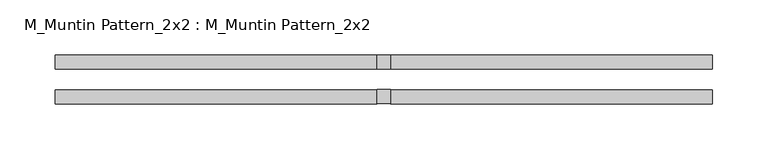
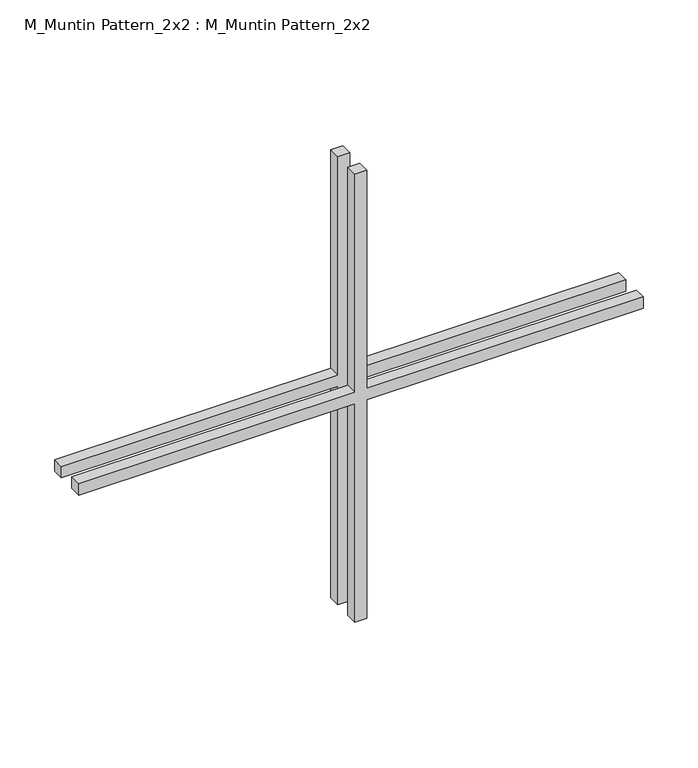
"""IFC4 building model written with IfcOpenShell, lengths in millimetres: proxy geometry, M_Muntin Pattern_2x2 : M_Muntin Pattern_2x2."""

from ifc_helpers import new_model, si_unit, frame, origin, place, context, project, spatial, polyline, outline, extrude, source, transform, mapped, element, save


def m_muntin_pattern_2x2_m_muntin_pattern_2x2_aaec3afb(model_context):
    return source(origin(), model_context, "Body", "SweptSolid", [
        extrude(outline(polyline([(257.1375, -6.35), (257.1375, -298.8), (244.4375, -298.8), (244.4375, -6.35), (0.0, -6.35), (0.0, 6.35), (244.4375, 6.35), (244.4375, 298.8), (257.1375, 298.8), (257.1375, 6.35), (501.575, 6.35), (501.575, -6.35), (257.1375, -6.35)])), frame((0.0, 9.525, 0.0), z_axis=(0.0, 1.0, 0.0), x_axis=(0.0, 0.0, 1.0)), (0.0, 0.0, 1.0), 12.7),
        extrude(outline(polyline([(257.1375, -6.35), (257.1375, -298.8), (244.4375, -298.8), (244.4375, -6.35), (0.0, -6.35), (0.0, 6.35), (244.4375, 6.35), (244.4375, 298.8), (257.1375, 298.8), (257.1375, 6.35), (501.575, 6.35), (501.575, -6.35), (257.1375, -6.35)])), frame((0.0, -22.225, 0.0), z_axis=(0.0, 1.0, 0.0), x_axis=(0.0, 0.0, 1.0)), (0.0, 0.0, 1.0), 12.7),
    ])


if __name__ == "__main__":
    model = new_model("IFC4")
    model_context = context("Model", 3, world=origin())
    ifc_project = project(units=[si_unit("LENGTHUNIT", "METRE", prefix="MILLI")], contexts=[model_context])
    site = spatial("IfcSite", under=ifc_project)
    building = spatial("IfcBuilding", under=site)
    placement = place(None, origin())
    m_muntin_pattern_2x2_m_muntin_pattern_2x2_shape = m_muntin_pattern_2x2_m_muntin_pattern_2x2_aaec3afb(model_context)
    element("IfcBuildingElementProxy", 1, Name="M_Muntin Pattern_2x2 : M_Muntin Pattern_2x2", ObjectType="M_Muntin Pattern_2x2 : M_Muntin Pattern_2x2", at=placement, inside=building, context=model_context, shape_type="MappedRepresentation", body=[
        mapped(m_muntin_pattern_2x2_m_muntin_pattern_2x2_shape, transform((0.0, 0.0, 0.0), x_axis=(1.0, 0.0, 0.0), y_axis=(0.0, 1.0, 0.0), z_axis=(0.0, 0.0, 1.0))),
    ])
    save(model, "model.ifc")

# Revit data of these elements
# Type "M_Muntin Pattern_2x2 : M_Muntin Pattern_2x2"
#   Width [instance default] = 1200 mm
#   Thickness = 12.7 mm
#   Height [instance default] = 1200 mm
#   Distance = 19.05 mm
#   Interior Material [instance default] = none
#   Exterior Material [instance default] = none
#   Default Elevation = 0
# Element 1 (IfcBuildingElementProxy, "M_Muntin Pattern_2x2 : M_Muntin Pattern_2x2")
#   Width = 597.6 mm
#   Height = 501.575 mm
#   Interior Material = Wood - Stained
#   Exterior Material = Clad - White
#   Materials on its faces: "Clad - White", "Wood - Stained"
# Materials
#   "Clad - White": class "Wood", colour RGB 242 242 238, transparency 0, Cost = 0
#   "Wood - Stained": class "Wood", colour RGB 227 170 128, transparency 0, Cost = 0
